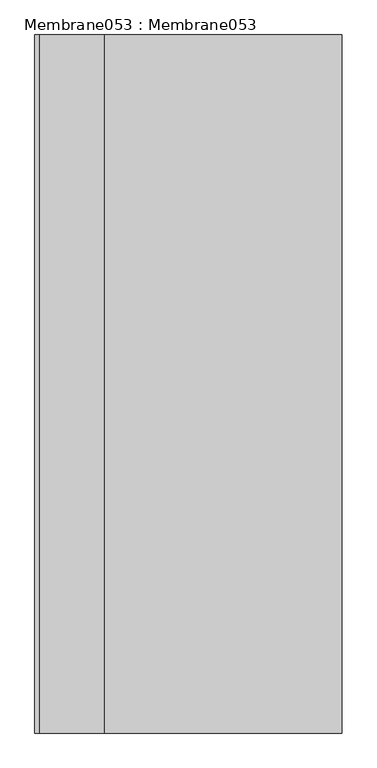
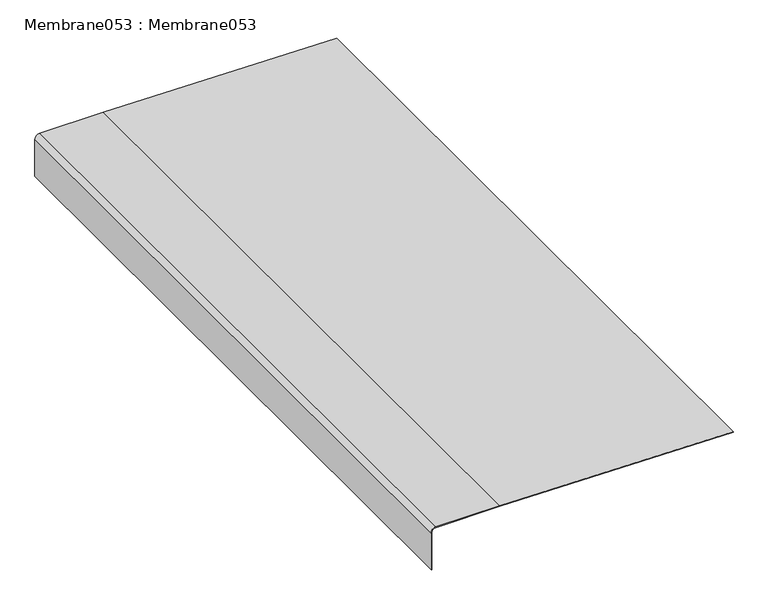
"""IFC4 building model written with IfcOpenShell, lengths in millimetres: proxy geometry, Membrane053 : Membrane053."""

from ifc_helpers import new_model, si_unit, point, frame, frame_2d, origin, place, context, project, spatial, polyline, circle_curve, trimmed, segment, composite_curve, outline, extrude, source, transform, mapped, element, save


def membrane053_membrane053_9e159549(model_context):
    return source(origin(), model_context, "Body", "SweptSolid", [
        extrude(outline(composite_curve([segment(trimmed(circle_curve(frame_2d((40234.5370749, -2761.211855)), 12.0), [point((40234.5370749, -2773.211855))], [point((40246.5370749, -2761.211855))], True, "CARTESIAN"), True, "CONTINUOUS"), segment(polyline([(40246.5370749, -2761.211855), (40246.5370749, -2575.7595485), (40236.7392216, -1894.9487955), (40238.7390146, -1894.9200155), (40248.5370749, -2575.7451577), (40248.5370749, -2761.211855)]), True, "CONTINUOUS"), segment(trimmed(circle_curve(frame_2d((40234.5370749, -2761.211855)), 14.0), [point((40248.5370749, -2761.211855))], [point((40234.5370749, -2775.211855))], False, "CARTESIAN"), True, "CONTINUOUS"), segment(polyline([(40234.5370749, -2775.211855), (40120.9129128, -2775.211855), (40120.9129128, -2773.211855), (40234.5370749, -2773.211855)]), True, "CONTINUOUS")], self_intersect=False)), frame((0.0, -1052.8906574, 0.0), z_axis=(0.0, 1.0, 0.0), x_axis=(0.0, 0.0, 1.0)), (0.0, 0.0, 1.0), 2000.0),
    ])


if __name__ == "__main__":
    model = new_model("IFC4")
    model_context = context("Model", 3, world=origin())
    ifc_project = project(units=[si_unit("LENGTHUNIT", "METRE", prefix="MILLI")], contexts=[model_context])
    site = spatial("IfcSite", under=ifc_project)
    building = spatial("IfcBuilding", under=site)
    placement = place(None, origin())
    membrane053_membrane053_shape = membrane053_membrane053_9e159549(model_context)
    element("IfcBuildingElementProxy", 1, Name="Membrane053 : Membrane053", ObjectType="Membrane053 : Membrane053", at=placement, inside=building, context=model_context, shape_type="MappedRepresentation", body=[
        mapped(membrane053_membrane053_shape, transform((0.0, 0.0, 0.0), x_axis=(1.0, 0.0, 0.0), y_axis=(0.0, 1.0, 0.0), z_axis=(0.0, 0.0, 1.0))),
    ])
    save(model, "model.ifc")

# Revit data of these elements
# Type "Membrane053 : Membrane053"
#   NameOverride = "Membrane053"
# Element 1 (IfcBuildingElementProxy, "Membrane053 : Membrane053")
#   Materials on its faces: "THREE PLY BUILT UP ROOF MEMBRANE"
# Materials
#   "THREE PLY BUILT UP ROOF MEMBRANE": class "Unassigned", colour RGB 63 63 63, transparency 0
